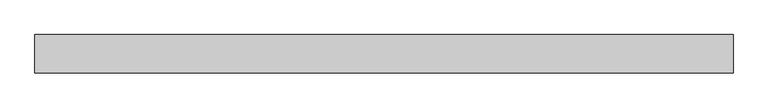
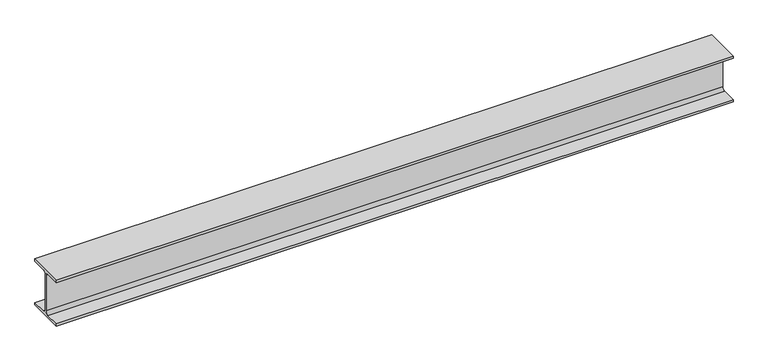
"""IFC4 building model written with IfcOpenShell, lengths in millimetres: beam geometry, 0912_Steel Framing_H-KSD3502 : H_SB_ASB_H-194x150x6x9."""

from ifc_helpers import new_model, si_unit, point, frame, frame_2d, origin, place, context, project, spatial, polyline, circle_curve, trimmed, segment, composite_curve, outline, extrude, source, transform, mapped, element, save


def beam_7a399356(model_context):
    return source(origin(), model_context, "Body", "SweptSolid", [
        extrude(outline(composite_curve([segment(polyline([(-75.0, -88.0), (-16.0, -88.0)]), True, "CONTINUOUS"), segment(trimmed(circle_curve(frame_2d((-16.0, -75.0)), 13.0), [point((-16.0, -88.0))], [point((-3.0, -75.0))], True, "CARTESIAN"), True, "CONTINUOUS"), segment(polyline([(-3.0, -75.0), (-3.0, 75.0)]), True, "CONTINUOUS"), segment(trimmed(circle_curve(frame_2d((-16.0, 75.0)), 13.0), [point((-3.0, 75.0))], [point((-16.0, 88.0))], True, "CARTESIAN"), True, "CONTINUOUS"), segment(polyline([(-16.0, 88.0), (-75.0, 88.0), (-75.0, 97.0), (75.0, 97.0), (75.0, 88.0), (16.0, 88.0)]), True, "CONTINUOUS"), segment(trimmed(circle_curve(frame_2d((16.0, 75.0)), 13.0), [point((16.0, 88.0))], [point((3.0, 75.0))], True, "CARTESIAN"), True, "CONTINUOUS"), segment(polyline([(3.0, 75.0), (3.0, -75.0)]), True, "CONTINUOUS"), segment(trimmed(circle_curve(frame_2d((16.0, -75.0)), 13.0), [point((3.0, -75.0))], [point((16.0, -88.0))], True, "CARTESIAN"), True, "CONTINUOUS"), segment(polyline([(16.0, -88.0), (75.0, -88.0), (75.0, -97.0), (-75.0, -97.0), (-75.0, -88.0)]), True, "CONTINUOUS")], self_intersect=False)), frame((-1579.8617116, 0.0, 0.0), z_axis=(1.0, 0.0, 0.0), x_axis=(0.0, 1.0, 0.0)), (0.0, 0.0, 1.0), 2719.057388),
    ])


if __name__ == "__main__":
    model = new_model("IFC4")
    model_context = context("Model", 3, world=origin())
    ifc_project = project(units=[si_unit("LENGTHUNIT", "METRE", prefix="MILLI")], contexts=[model_context])
    site = spatial("IfcSite", under=ifc_project)
    building = spatial("IfcBuilding", under=site)
    placement = place(None, origin())
    beam_shape = beam_7a399356(model_context)
    element("IfcBeam", 1, ObjectType="0912_Steel Framing_H-KSD3502 : H_SB_ASB_H-194x150x6x9", at=placement, inside=building, context=model_context, shape_type="MappedRepresentation", body=[
        mapped(beam_shape, transform((0.0, 0.0, 0.0), x_axis=(1.0, 0.0, 0.0), y_axis=(0.0, 1.0, 0.0), z_axis=(0.0, 0.0, 1.0))),
    ])
    save(model, "model.ifc")

# Revit data of these elements
# Type "0912_Steel Framing_H-KSD3502 : H_SB_ASB_H-194x150x6x9"
#   H_WM Code_1 = "S01AA002-00001 | Main Steel Structure Fabrication Work | Shelter/Building | Medium Steel - Standard (90KG/M>Weight≥30KG/M) | Material: (   )"
#   H_WM Code_2 = "S03AA028-00001 | Main Steel Structure Erection Work | Shelter/Building | Medium Steel (90KG/M>Weight≥30KG/M) | Material: (   )"
#   H_WM Code_3 = "S01AA010-00001 | Main Steel Structure Fabrication Work | Shelter/Building | Steel Painting/Coating | for Non-Fireproofed Steel Surface, Surface Preparation, Primer, Second & Final Coat | Material: (   )"
#   H_Q'ty Cal Type Tag = "SB-Q2"
#   Width = 15.0 cm
#   Web Thickness = 0.6 cm
#   Web Fillet = 1.3 cm
#   Warping Constant = 43316.0 cm⁶
#   W = 0
#   Torsional Moment of Inertia = 8.622 cm⁴
#   Section Area = 39.01 cm²
#   Plastic Modulus weak axis = 104.0 cm³
#   Plastic Modulus strong axis = 309.0 cm³
#   Perimeter = 0.95 m²/m
#   Nominal Weight = 30.60 kgf/m
#   Moment of Inertia weak axis = 507.00 cm⁴
#   Moment of Inertia strong axis = 2690.00 cm⁴
#   Height = 19.4 cm
#   Flange Thickness = 0.9 cm
#   Elastic Modulus weak axis = 67.6 cm³
#   Elastic Modulus strong axis = 277.0 cm³
#   Centroid Vertical = 9.7 cm
#   Centroid Horizontal = 7.5 cm
#   Ix = 26900000
#   Length [instance default] = 1.5240 m
#   Zx = 309000
#   b = 0.1500 m
#   h = 0.1940 m
#   r = 0.0130 m
#   s = 0.0060 m
#   t = 0.0090 m
#   A = 0.003901 m²
#   Structural Material [instance default] = Steel, 45-345
#   Assembly Code = ""
# Element 1 (IfcBeam, "0912_Steel Framing_H-KSD3502 : H_SB_ASB_H-194x150x6x9")
#   Structural Material = none
# Materials
#   "Steel, 45-345": class "Metal", colour RGB 189 187 185, transparency 0, Description = "Steel 345 MPa", Cost = 0
